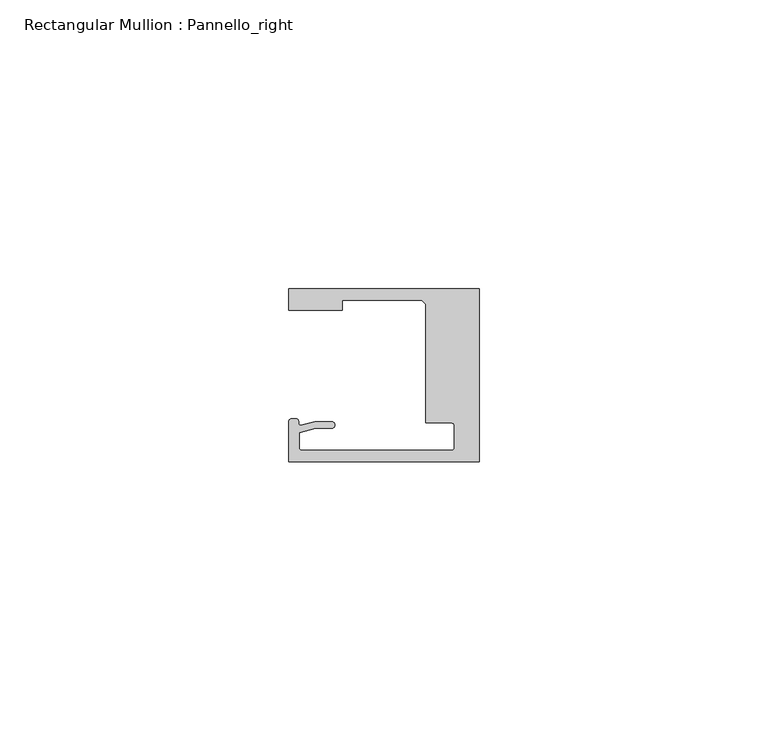
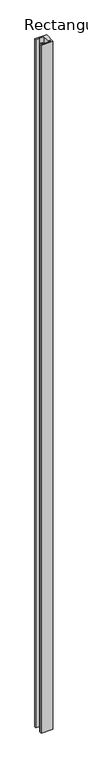
"""IFC4 building model written with IfcOpenShell, lengths in millimetres: member geometry, Rectangular Mullion : Pannello_right."""

from ifc_helpers import new_model, si_unit, frame, origin, place, context, project, spatial, polyline, circle_curve, source, transform, mapped, element, save
from ifc_brep_helpers import plane_surface, cylinder_surface, revolved_surface, extruded_surface, spline_curve, advanced_brep


def rectangular_mullion_pannello_right_d39bb4b2(model_context):
    return source(origin(), model_context, "Body", "AdvancedBrep", [
        advanced_brep(
        [(-33.0, 15.0, 0.0), (-33.0, 11.3000004, 0.0), (-23.700041, 11.3000004, 0.0), (-23.700041, 13.0000004, 0.0), (-10.0000103, 13.0000004, 0.0), (-9.2999726, 12.2999849, 0.0), (-9.2999726, -8.2500595, 0.0), (-4.7999726, -8.2500595, 0.0), (-4.2999726, -8.7500595, 0.0), (-4.2999726, -12.50001, 0.0), (-4.7999726, -13.00001, 0.0), (-30.69998, -13.00001, 0.0), (-31.19998, -12.50001, 0.0), (-31.19998, -9.9657591, 0.0), (-28.3419477, -9.1999523, 0.0), (-25.59998, -9.1999523, 0.0), (-25.59998, -7.9999523, 0.0), (-28.4999305, -7.9999523, 0.0), (-30.9223017, -8.6490241, 0.0), (-33.0000135, -8.0000472, 0.0), (-33.0000135, -15.0, 0.0), (0.0, -15.0, 0.0), (0.0, 15.0, 0.0), (-33.0, 15.0, -2026.9999865), (0.0, 15.0, -2026.9999865), (0.0, -15.0, -2026.9999865), (-33.0000135, -15.0, -2026.9999865), (-33.0000135, -8.0000472, -2026.9999865), (-30.9223017, -8.6490241, -2026.9999865), (-28.4999305, -7.9999523, -2026.9999865), (-25.59998, -7.9999523, -2026.9999865), (-25.59998, -9.1999523, -2026.9999865), (-28.3419477, -9.1999523, -2026.9999865), (-31.19998, -9.9657591, -2026.9999865), (-31.19998, -12.50001, -2026.9999865), (-30.69998, -13.00001, -2026.9999865), (-4.7999726, -13.00001, -2026.9999865), (-4.2999726, -12.50001, -2026.9999865), (-4.2999726, -8.7500595, -2026.9999865), (-4.7999726, -8.2500595, -2026.9999865), (-9.2999726, -8.2500595, -2026.9999865), (-9.2999726, 12.2999849, -2026.9999865), (-10.0000103, 13.0000004, -2026.9999865), (-23.700041, 13.0000004, -2026.9999865), (-23.700041, 11.3000004, -2026.9999865), (-33.0, 11.3000004, -2026.9999865)],
        [
            (0, 1),
            (1, 2),
            (2, 3),
            (3, 4),
            (4, 5),
            (5, 6),
            (6, 7),
            (7, 8, circle_curve(frame((-4.7999726, -8.7500595, 0.0), z_axis=(0.0, 0.0, -1.0), x_axis=(0.0, 1.0, 0.0)), 0.5)),
            (8, 9),
            (9, 10, circle_curve(frame((-4.7999726, -12.50001, 0.0), z_axis=(0.0, 0.0, -1.0), x_axis=(1.0, 0.0, 0.0)), 0.5)),
            (10, 11),
            (11, 12, circle_curve(frame((-30.69998, -12.50001, 0.0), z_axis=(0.0, 0.0, -1.0), x_axis=(0.0, -1.0, 0.0)), 0.5)),
            (12, 13),
            (13, 14),
            (14, 15),
            (15, 16, circle_curve(frame((-25.59998, -8.5999523, 0.0), z_axis=(0.0, 0.0, 1.0), x_axis=(0.0, -1.0, 0.0)), 0.6)),
            (16, 17),
            (17, 18),
            (18, 19, spline_curve(3, [(-30.9223017, -8.6490241, 0.0), (-31.312054066, -8.717747958, 0.0), (-31.298563602, -8.366228555, 0.0), (-31.305645054, -7.690065204, 0.0), (-31.357433266, -7.563996614, 0.0), (-32.262327879, -7.456527435, 0.0), (-33.0000135, -7.457047519, 0.0), (-33.0000135, -8.0000472, 0.0)], [4, 2, 2, 4], [0.0, 0.001840817752199412, 0.004996616814974408, 0.007702013405570312])),
            (19, 20),
            (20, 21),
            (21, 22),
            (22, 0),
            (23, 24),
            (24, 25),
            (25, 26),
            (26, 27),
            (27, 28, spline_curve(3, [(-33.0000135, -8.0000472, -2026.9999865), (-33.0000135, -7.457047519, -2026.9999865), (-32.262327879, -7.456527435, -2026.9999865), (-31.357433266, -7.563996614, -2026.9999865), (-31.305645054, -7.690065204, -2026.9999865), (-31.298563602, -8.366228555, -2026.9999865), (-31.312054066, -8.717747958, -2026.9999865), (-30.9223017, -8.6490241, -2026.9999865)], [4, 2, 2, 4], [0.0, 0.0027053965905959043, 0.0058611956533709, 0.007702013405570312])),
            (28, 29),
            (29, 30),
            (30, 31, circle_curve(frame((-25.59998, -8.5999523, -2026.9999865), z_axis=(0.0, 0.0, -1.0), x_axis=(0.0, -1.0, 0.0)), 0.6)),
            (31, 32),
            (32, 33),
            (33, 34),
            (34, 35, circle_curve(frame((-30.69998, -12.50001, -2026.9999865), z_axis=(0.0, 0.0, 1.0), x_axis=(0.0, -1.0, 0.0)), 0.5)),
            (35, 36),
            (36, 37, circle_curve(frame((-4.7999726, -12.50001, -2026.9999865), z_axis=(0.0, 0.0, 1.0), x_axis=(1.0, 0.0, 0.0)), 0.5)),
            (37, 38),
            (38, 39, circle_curve(frame((-4.7999726, -8.7500595, -2026.9999865), z_axis=(0.0, 0.0, 1.0), x_axis=(0.0, 1.0, 0.0)), 0.5)),
            (39, 40),
            (40, 41),
            (41, 42),
            (42, 43),
            (43, 44),
            (44, 45),
            (45, 23),
            (0, 23),
            (45, 1),
            (44, 2),
            (43, 3),
            (42, 4),
            (41, 5),
            (40, 6),
            (39, 7),
            (38, 8),
            (37, 9),
            (36, 10),
            (35, 11),
            (34, 12),
            (33, 13),
            (32, 14),
            (31, 15),
            (30, 16),
            (29, 17),
            (28, 18),
            (27, 19),
            (26, 20),
            (25, 21),
            (24, 22),
        ],
        [
            plane_surface(frame((0.0, -36.2491502, 0.0), z_axis=(0.0, 0.0, 1.0), x_axis=(-1.0, 0.0, 0.0))),
            plane_surface(frame((0.0, -36.2491502, -2026.9999865), z_axis=(0.0, 0.0, -1.0), x_axis=(-1.0, 0.0, 0.0))),
            plane_surface(frame((-33.0, 15.0, 0.0), z_axis=(-1.0, 0.0, 0.0), x_axis=(0.0, 0.0, -1.0))),
            plane_surface(frame((-33.0, 11.3000004, 0.0), z_axis=(0.0, -1.0, 0.0), x_axis=(0.0, 0.0, -1.0))),
            plane_surface(frame((-23.700041, 11.3000004, 0.0), z_axis=(1.0, 0.0, 0.0), x_axis=(0.0, 0.0, -1.0))),
            plane_surface(frame((-23.700041, 13.0000004, 0.0), z_axis=(0.0, -1.0, 0.0), x_axis=(0.0, 0.0, -1.0))),
            plane_surface(frame((-10.0000103, 13.0000004, 0.0), z_axis=(-0.7070955486278075, -0.7071180135668587, 0.0), x_axis=(0.0, 0.0, -1.0))),
            plane_surface(frame((-9.2999726, 12.2999849, 0.0), z_axis=(-1.0, 0.0, 0.0), x_axis=(0.0, 0.0, -1.0))),
            plane_surface(frame((-9.2999726, -8.2500595, 0.0), z_axis=(0.0, -1.0, 0.0), x_axis=(0.0, 0.0, -1.0))),
            revolved_surface(polyline([(-4.7999726, -8.2500595, -2026.9999865), (-4.7999726, -8.2500595, 0.0)]), (-4.7999726, -8.7500595, 0.0), (0.0, 0.0, -1.0)),
            plane_surface(frame((-4.2999726, -8.7500595, 0.0), z_axis=(-1.0, 0.0, 0.0), x_axis=(0.0, 0.0, -1.0))),
            revolved_surface(polyline([(-4.2999726, -12.50001, -2026.9999865), (-4.2999726, -12.50001, 0.0)]), (-4.7999726, -12.50001, 0.0), (0.0, 0.0, -1.0)),
            plane_surface(frame((-4.7999726, -13.00001, 0.0), z_axis=(0.0, 1.0, 0.0), x_axis=(0.0, 0.0, -1.0))),
            revolved_surface(polyline([(-30.69998, -13.00001, -2026.9999865), (-30.69998, -13.00001, 0.0)]), (-30.69998, -12.50001, 0.0), (0.0, 0.0, -1.0)),
            plane_surface(frame((-31.19998, -12.50001, 0.0), z_axis=(1.0, 0.0, 0.0), x_axis=(0.0, 0.0, -1.0))),
            plane_surface(frame((-31.19998, -9.9657591, 0.0), z_axis=(0.2588188320428738, -0.9659258833782035, 0.0), x_axis=(0.0, 0.0, -1.0))),
            plane_surface(frame((-28.3419477, -9.1999523, 0.0), z_axis=(0.0, -1.0, 0.0), x_axis=(0.0, 0.0, -1.0))),
            cylinder_surface(frame((-25.59998, -8.5999523, 0.0), z_axis=(0.0, 0.0, 1.0), x_axis=(0.0, -1.0, 0.0)), 0.6),
            plane_surface(frame((-25.59998, -7.9999523, 0.0), z_axis=(0.0, 1.0, 0.0), x_axis=(0.0, 0.0, -1.0))),
            plane_surface(frame((-28.4999305, -7.9999523, 0.0), z_axis=(-0.2588188320019168, 0.965925883389178, 0.0), x_axis=(0.0, 0.0, -1.0))),
            extruded_surface(spline_curve(3, [(-30.9223017, -8.6490241, -2026.9999865), (-31.312054066, -8.717747958, -2026.9999865), (-31.298563602, -8.366228555, -2026.9999865), (-31.305645054, -7.690065204, -2026.9999865), (-31.357433266, -7.563996614, -2026.9999865), (-32.262327879, -7.456527435, -2026.9999865), (-33.0000135, -7.457047519, -2026.9999865), (-33.0000135, -8.0000472, -2026.9999865)], [4, 2, 2, 4], [0.0, 0.001840817752199412, 0.004996616814974408, 0.007702013405570312]), (0.0, 0.0, 2026.9999865), 2026.9999865),
            plane_surface(frame((-33.0000135, -8.0000472, 0.0), z_axis=(-1.0, 0.0, 0.0), x_axis=(0.0, 0.0, -1.0))),
            plane_surface(frame((-33.0000135, -15.0, 0.0), z_axis=(0.0, -1.0, 0.0), x_axis=(0.0, 0.0, -1.0))),
            plane_surface(frame((0.0, -15.0, 0.0), z_axis=(1.0, 0.0, 0.0), x_axis=(0.0, 0.0, -1.0))),
            plane_surface(frame((0.0, 15.0, 0.0), z_axis=(0.0, 1.0, 0.0), x_axis=(0.0, 0.0, -1.0))),
        ],
        [
            (0, [[1, 2, 3, 4, 5, 6, 7, 8, 9, 10, 11, 12, 13, 14, 15, 16, 17, 18, 19, 20, 21, 22, 23]]),
            (1, [[24, 25, 26, 27, 28, 29, 30, 31, 32, 33, 34, 35, 36, 37, 38, 39, 40, 41, 42, 43, 44, 45, 46]]),
            (2, [[-1, 47, -46, 48]]),
            (3, [[-2, -48, -45, 49]]),
            (4, [[-3, -49, -44, 50]]),
            (5, [[-4, -50, -43, 51]]),
            (6, [[-5, -51, -42, 52]]),
            (7, [[-6, -52, -41, 53]]),
            (8, [[-7, -53, -40, 54]]),
            (9, [[-8, -54, -39, 55]]),
            (10, [[-9, -55, -38, 56]]),
            (11, [[-10, -56, -37, 57]]),
            (12, [[-11, -57, -36, 58]]),
            (13, [[-12, -58, -35, 59]]),
            (14, [[-13, -59, -34, 60]]),
            (15, [[-14, -60, -33, 61]]),
            (16, [[-15, -61, -32, 62]]),
            (17, [[-16, -62, -31, 63]]),
            (18, [[-17, -63, -30, 64]]),
            (19, [[-18, -64, -29, 65]]),
            (20, [[-19, -65, -28, 66]]),
            (21, [[-20, -66, -27, 67]]),
            (22, [[-21, -67, -26, 68]]),
            (23, [[-22, -68, -25, 69]]),
            (24, [[-23, -69, -24, -47]]),
        ],
    ),
    ])


if __name__ == "__main__":
    model = new_model("IFC4")
    model_context = context("Model", 3, world=origin())
    ifc_project = project(units=[si_unit("LENGTHUNIT", "METRE", prefix="MILLI")], contexts=[model_context])
    site = spatial("IfcSite", under=ifc_project)
    building = spatial("IfcBuilding", under=site)
    placement = place(None, origin())
    rectangular_mullion_pannello_right_shape = rectangular_mullion_pannello_right_d39bb4b2(model_context)
    element("IfcMember", 1, ObjectType="Rectangular Mullion : Pannello_right", at=placement, inside=building, context=model_context, shape_type="MappedRepresentation", body=[
        mapped(rectangular_mullion_pannello_right_shape, transform((0.0, 0.0, 0.0), x_axis=(1.0, 0.0, 0.0), y_axis=(0.0, 1.0, 0.0), z_axis=(0.0, 0.0, 1.0))),
    ])
    save(model, "model.ifc")

# Revit data of these elements
# Type "Rectangular Mullion : Pannello_right"
#   built-in parameter 1007322 = 0.0984252 (stored number, unit not read)
#   built-in parameter 1007321 = 0.0305117 (stored number, unit not read)
#   built-in parameter 1007320 = 0 (stored number, unit not read)
